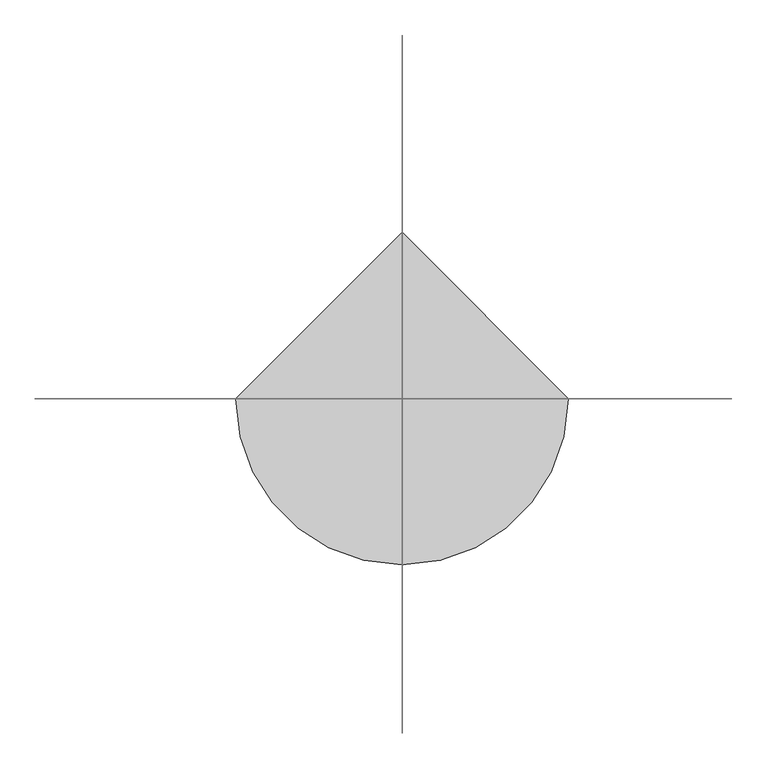
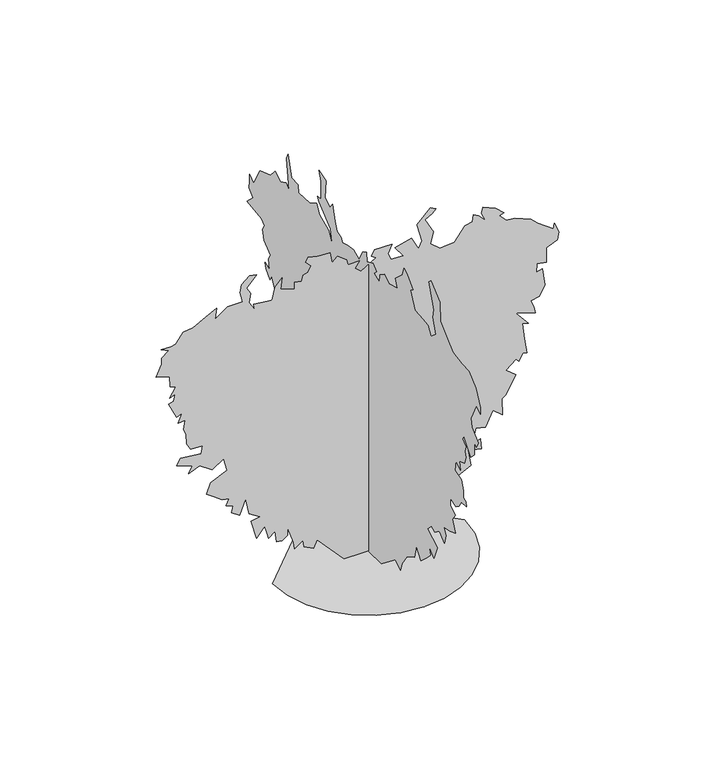
"""IFC4 building model written with IfcOpenShell, lengths in millimetres: proxy geometry, meadowlark 26084 : meadowlark 26084."""

from ifc_helpers import new_model, si_unit, origin, place, context, project, spatial, triangles, source, transform, mapped, element, save


def entourage_9ef344a8(model_context):
    return source(origin(), model_context, "Body", "Tessellation", [
        triangles([(-63.9369313, 2.6e-06, 2.5813025), (-98.6351404, 1.9e-06, 41.3616468), (-133.3335948, 1.1e-06, 80.1421467), (-143.538813, 2.7e-06, 59.7314513), (-168.0315495, 3.1e-06, 71.9778149), (-170.0726858, 2.1e-06, 90.347365), (-192.5245312, 3.9e-06, 76.0598514), (-194.5656857, 2.9e-06, 94.4296558), (-210.8940858, 9e-07, 139.3333375), (-210.8940858, 2.1e-06, 118.9223832), (-225.1818402, 3.4e-06, 108.7171649), (-239.469104, 3.9e-06, 110.7583103), (-243.5513948, 2.2e-06, 141.3742286), (-260.2917792, 3.7e-06, 128.4682213), (-264.2033864, 3e-06, 143.1357217), (-270.0860397, 2e-06, 163.8260649), (-290.4949502, 4.4e-06, 139.3333375), (-304.7824684, 2e-06, 190.3599468), (-282.331386, 8e-07, 194.4422376), (-310.9064223, 9e-07, 212.8117922), (-319.0699865, -1.4e-06, 257.7162279), (-335.3996584, 1.7e-06, 216.894083), (-355.8110942, 1.8e-06, 231.181583), (-351.7293303, 5e-07, 249.5511376), (-370.0986305, 9e-07, 255.674056), (-361.9325229, -4e-07, 272.003746), (-380.3043303, 2e-07, 276.0855281), (-401.9400736, 2e-07, 291.703997), (-421.1247311, 3e-07, 304.6605463), (-410.918995, -1.9e-06, 333.2355826), (-368.1987102, -4.9e-06, 351.9401459), (-376.2200229, -6.6e-06, 386.3038187), (-406.8371947, -4.1e-06, 367.9345184), (-439.493995, -4.1e-06, 390.385619), (-468.0690313, -2.1e-06, 378.137711), (-457.8632953, -3.5e-06, 394.4673829), (-498.6862032, -2.7e-06, 410.7970548), (-488.4805035, -4.1e-06, 427.1242195), (-435.4122311, -6.1e-06, 421.0002474), (-431.3304308, -7.5e-06, 441.4117195), (-461.9450955, -6.2e-06, 443.4538914), (-472.1508316, -6.9e-06, 461.8231553), (-474.1929671, -8.4e-06, 488.3560198), (-480.3169393, -9e-06, 502.6435561), (-476.2325955, -1.06e-05, 527.1367922), (-495.4832737, -9.7e-06, 526.35192), (-484.3987032, -1.16e-05, 549.5878564), (-498.6862032, -1.06e-05, 543.466464), (-519.0951319, -1.23e-05, 586.3290004), (-506.8497674, -1.3e-05, 590.4107643), (-502.7680035, -1.43e-05, 608.7800646), (-517.0555035, -1.33e-05, 602.6561288), (-500.7258316, -1.55e-05, 627.1493649), (-516.1995237, -1.52e-05, 634.2689884), (-517.0555035, -1.68e-05, 661.848337), (-551.7544756, -1.59e-05, 672.0540367), (-537.4644321, -1.84e-05, 702.6687378), (-538.1857907, -1.94e-05, 720.3319038), (-519.0951319, -2.1e-05, 733.2859097), (-539.506604, -2.07e-05, 743.4916094), (-512.7375257, -2.18e-05, 742.0895147), (-500.7258316, -2.25e-05, 745.5312378), (-482.3565313, -2.49e-05, 772.0666094), (-455.8236669, -2.62e-05, 774.1062378), (-423.1668666, -2.87e-05, 792.4755381), (-395.1176339, -3.08e-05, 806.3871162), (-398.6736305, -2.9e-05, 778.1880381), (-366.0168303, -3.17e-05, 800.6416821), (-327.2360942, -3.34e-05, 800.6416821), (-334.4166515, -3.47e-05, 827.9339842), (-330.1088113, -3.62e-05, 849.0616917), (-308.8667939, -3.81e-05, 865.9552826), (-290.4949502, -3.87e-05, 861.8734823), (-317.5358142, -3.58e-05, 834.0731443), (-306.8246221, -3.53e-05, 816.9688105), (-310.9064223, -3.36e-05, 792.4755381), (-296.6189042, -3.29e-05, 770.0245102), (-298.6610579, -3.37e-05, 784.3120102), (-251.0357672, -3.54e-05, 778.383593), (-243.5513948, -3.77e-05, 810.8473818), (-225.1818402, -3.97e-05, 831.2563105), (-228.2958943, -3.78e-05, 801.312208), (-192.5245312, -3.86e-05, 788.3937378), (-192.5245312, -3.97e-05, 806.7630381), (-173.5245645, -4.03e-05, 803.1613684), (-170.0726858, -4.14e-05, 819.0109823), (-157.8260678, -4.22e-05, 823.0927099), (-149.662004, -4.34e-05, 837.3802826), (-163.9495131, -4.36e-05, 851.6677826), (-157.8260678, -4.46e-05, 863.9131107), (-131.292195, -4.54e-05, 857.7916821), (-100.6760314, -4.66e-05, 855.7495102), (-94.5528496, -4.52e-05, 827.1745102), (-80.2653314, -4.65e-05, 839.4223818), (-56.9158573, -4.65e-05, 821.1673914), (-53.7314587, -4.57e-05, 806.7630381), (-23.1153655, -4.71e-05, 806.7630381), (-35.3616542, -4.56e-05, 790.4359097), (-19.0331746, -4.54e-05, 776.1484097), (19.7470164, -4.86e-05, 800.6416821), (7.5007532, -4.85e-05, 808.8052099), (15.1231208, -4.98e-05, 823.890263), (60.5683824, -5.17e-05, 823.0927099), (50.5958261, -4.99e-05, 799.816151), (58.5274868, -4.92e-05, 782.2723818), (91.1845505, -5.05e-05, 780.2302099), (68.732964, -5.13e-05, 810.8473818), (111.5952414, -5.38e-05, 821.0506107), (129.9650504, -5.25e-05, 786.3541821), (138.9452253, -5.4e-05, 804.6625122), (125.8830048, -5.64e-05, 853.7099545), (160.581223, -6e-05, 888.4063831), (174.868723, -6.01e-05, 880.2427826), (164.6635138, -5.91e-05, 870.0370829), (146.2937048, -5.76e-05, 859.8313105), (168.7455503, -5.62e-05, 819.0109823), (161.0930195, -5.4e-05, 788.6985884), (185.0742047, -5.39e-05, 767.9848818), (203.4434868, -5.48e-05, 770.0245102), (223.8544503, -5.58e-05, 772.0666094), (250.3885683, -5.9e-05, 806.7630381), (269.7101179, -6.01e-05, 811.2766434), (272.8393963, -6.13e-05, 829.2166821), (285.0872861, -6.15e-05, 823.0927099), (304.0839645, -6.12e-05, 803.1613684), (293.2508503, -6.21e-05, 827.1745102), (297.3326324, -6.31e-05, 841.4620102), (329.9894508, -6.37e-05, 827.1745102), (351.394031, -6.35e-05, 807.9441433), (340.0529354, -6.27e-05, 803.4457987), (358.5644508, -6.24e-05, 784.3120102), (381.0180948, -6.33e-05, 782.2723818), (422.1051581, -6.41e-05, 765.7470823), (440.2077596, -6.38e-05, 747.5734097), (481.0306675, -6.39e-05, 718.9984097), (483.0702959, -6.48e-05, 733.2859097), (495.3181675, -6.36e-05, 704.710837), (491.2364036, -6.23e-05, 684.2994375), (462.6588238, -6.03e-05, 672.0540367), (462.6588238, -5.8e-05, 633.273337), (438.1681312, -5.71e-05, 637.3550646), (436.1259593, -5.57e-05, 614.9040367), (452.4556312, -5.67e-05, 618.9857643), (458.5770598, -5.41e-05, 572.041464), (444.2895235, -5.19e-05, 545.5060925), (421.8384593, -5.07e-05, 541.4242922), (430.0020235, -4.98e-05, 521.0128201), (434.0863309, -4.91e-05, 504.6856916), (383.0577232, -4.78e-05, 521.0128201), (415.7145235, -4.69e-05, 482.2346274), (399.3873951, -4.64e-05, 486.3163914), (405.5087874, -4.42e-05, 443.4538914), (411.6327232, -4.2e-05, 402.6309471), (401.4269872, -4.17e-05, 404.673119), (391.2212874, -4.01e-05, 386.3038187), (383.0577232, -4.03e-05, 394.4673829), (356.5248588, -3.79e-05, 374.0559471), (383.0577232, -3.77e-05, 351.6048466), (356.5248588, -3.39e-05, 306.7001747), (346.3191227, -3.29e-05, 298.5365923), (348.3587511, -3.03e-05, 253.6334284), (323.4463909, -3.05e-05, 274.9933165), (303.4565864, -2.73e-05, 235.2636194), (278.9633503, -2.66e-05, 241.3868104), (266.8272088, -2.35e-05, 199.2829668), (291.2086966, -2.52e-05, 208.7297557), (293.2508503, -2.36e-05, 180.1547194), (258.5518782, -2.25e-05, 188.3190466), (266.7179858, -2.02e-05, 143.415374), (232.0187775, -1.77e-05, 127.0867195), (215.6903774, -1.54e-05, 100.5528377), (197.3205684, -1.5e-05, 106.6760195), (191.1973775, -1.2e-05, 61.7723423), (176.9098775, -1.3e-05, 88.306474), (150.3759956, -8.8e-06, 37.2796104), (132.0059414, -8.8e-06, 51.5671195), (68.732964, -3.2e-06, 2.5813025), (5e-07, 58.5086925, 0.0), (5.6e-06, 119.7410287, 55.1089), (6.1e-06, 137.5863239, 49.658565), (5.6e-06, 170.7679014, 104.0948725), (5.5e-06, 180.9731106, 91.8482545), (9.8e-06, 197.3017651, 73.4787044), (6.8e-06, 213.6304195, 87.7662181), (6.7e-06, 205.4660923, 93.8893999), (9.7e-06, 223.8356469, 144.9162635), (8.6e-06, 231.9999742, 112.2589454), (1e-05, 238.1231651, 136.7519272), (1.13e-05, 276.9033925, 128.5875999), (1.12e-05, 254.4523283, 148.9982999), (1.22e-05, 274.8637822, 151.0394453), (1.45e-05, 307.5205825, 171.4501453), (1.42e-05, 280.9851927, 191.8608363), (1.68e-05, 299.3544748, 232.6824725), (1.68e-05, 317.7263186, 214.3126635), (1.89e-05, 350.3043809, 228.0708535), (1.99e-05, 340.1773828, 261.2569819), (2.07e-05, 354.4649191, 265.338764), (2.22e-05, 356.5045112, 297.9955825), (2.36e-05, 393.2456552, 293.9138004), (2.61e-05, 411.6149554, 332.6945546), (2.58e-05, 397.3274554, 338.8184904), (2.92e-05, 438.1478199, 377.5992265), (2.82e-05, 405.4910196, 385.7627907), (2.9e-05, 411.6149554, 398.0081552), (2.55e-05, 417.7363478, 412.2956552), (2.48e-05, 395.2852836, 418.4196273), (2.73e-05, 415.6967194, 455.1581915), (2.98e-05, 436.1081915, 491.8993355), (2.95e-05, 444.2717557, 477.6118355), (3.11e-05, 460.5988841, 498.0207278), (3.2e-05, 466.7228199, 512.3082642), (3.07e-05, 446.3113841, 504.1447), (3.21e-05, 450.3956915, 530.6800715), (3.24e-05, 440.1899554, 547.0072), (3.47e-05, 470.8046202, 569.4583005), (3.61e-05, 476.928556, 595.9937084), (3.64e-05, 468.7649918, 610.2812084), (3.74e-05, 481.0103562, 622.5265366), (4.07e-05, 546.3265002, 630.6926805), (4.07e-05, 519.7910923, 657.2255087), (4.22e-05, 538.1603926, 673.5551805), (4.29e-05, 536.5677936, 692.1911797), (4.37e-05, 535.3943187, 712.0133709), (4.23e-05, 517.7489204, 698.0459095), (3.89e-05, 487.134292, 751.1141819), (3.76e-05, 440.1899554, 767.4438538), (3.77e-05, 419.7785196, 789.8948816), (3.6e-05, 395.2852836, 775.6073816), (3.55e-05, 370.7920475, 787.8553259), (3.44e-05, 358.546683, 775.6073816), (3.84e-05, 368.7524191, 857.250654), (3.88e-05, 362.6284833, 871.5382267), (3.56e-05, 346.2988114, 816.4303259), (3.43e-05, 317.7237751, 814.388154), (3.33e-05, 315.6841467, 793.9766819), (3.12e-05, 262.6158925, 798.0584822), (3.06e-05, 234.0411286, 814.388154), (2.9e-05, 219.7536105, 791.9370535), (2.65e-05, 180.9731106, 773.5677532), (2.43e-05, 162.603556, 740.9084095), (2.65e-05, 170.7679014, 783.7709822), (3.06e-05, 223.8356469, 824.5938538), (3.15e-05, 229.9590922, 836.8392546), (3.08e-05, 213.6301652, 838.8814264), (3.3e-05, 213.6301652, 887.8678986), (3.45e-05, 223.8356469, 912.3585548), (3.26e-05, 191.1785923, 902.1553986), (3.06e-05, 195.2606287, 853.1689264), (2.91e-05, 172.8087833, 840.9209822), (2.93e-05, 162.603556, 855.2085548), (2.71e-05, 150.356947, 816.4303259), (2.57e-05, 142.1926198, 793.9766819), (2.47e-05, 123.8230652, 787.8553259), (2.4e-05, 117.7001377, 777.6495535), (2.32e-05, 95.248047, 783.7709822), (2.23e-05, 68.7141651, 787.8553259), (2.06e-05, 43.1368564, 776.3617687), (2.13e-05, 25.8518877, 808.2641819), (2.09e-05, 9.5229755, 816.4303259), (1.98e-05, 7.4819061, 791.9370535), (1.91e-05, -19.0520211, 804.1824543), (1.78e-05, -35.3804508, 789.8948816), (1.78e-05, -25.1750781, 779.6891819), (1.63e-05, -49.6682165, 769.4834822), (1.72e-05, -51.7091075, 791.9370535), (1.69e-05, -72.1200574, 806.2245535), (1.54e-05, -92.5307528, 791.9370535), (1.42e-05, -129.2700982, 802.1428259), (1.56e-05, -121.105771, 824.5938538), (1.54e-05, -153.0015985, 852.691412), (1.61e-05, -159.8860075, 875.6199543), (1.52e-05, -172.1326437, 867.4564264), (1.28e-05, -200.7076618, 840.9209822), (1.3e-05, -188.4607894, 832.7574543), (1.02e-05, -208.8717347, 789.8948816), (8.5e-06, -245.6110801, 787.8553259), (7.4e-06, -268.0641973, 783.7709822), (5.8e-06, -280.3095436, 761.3198816), (5.7e-06, -303.1314609, 780.7331589), (8e-06, -290.5152796, 820.5121262), (8.8e-06, -294.5970617, 842.963154), (1.25e-05, -272.1459794, 906.2371988), (1.25e-05, -280.3095436, 914.4007267), (9.2e-06, -321.1299262, 879.7017546), (6.9e-06, -323.1720617, 828.675654), (4.3e-06, -354.6452497, 799.5291046), (2.2e-06, -380.3221344, 777.6495535), (1e-07, -421.1424989, 771.5255814), (-1.3e-06, -451.7596707, 769.4834822), (-3.9e-06, -482.3768789, 740.9084095), (-6.6e-06, -502.7857713, 700.0880814), (-7.4e-06, -502.7857713, 681.7187811), (-6e-06, -486.4586429, 696.0062811), (-2.7e-06, -459.9232349, 644.9801805), (-3.9e-06, -466.0472071, 624.5687084), (-6.3e-06, -494.6222071, 598.0333005), (-6.6e-06, -486.4586429, 581.7061721), (-5.9e-06, -476.2529068, 587.8301442), (-7.3e-06, -476.2529068, 555.1708005), (-7.3e-06, -459.9232349, 538.8436357), (-4.3e-06, -429.3086065, 577.6244081), (-4.5e-06, -423.1846707, 567.4186721), (-5.7e-06, -439.5143426, 555.1708005), (-6.2e-06, -433.3903705, 538.8436357), (-7.1e-06, -439.5143426, 524.5561357), (-7.6e-06, -431.3482349, 504.1447), (-7e-06, -408.8971344, 495.9810994), (-8.2e-06, -412.9789347, 473.5300352), (-6.6e-06, -392.5674625, 487.8175352), (-7.7e-06, -388.4856986, 459.2425352), (-9.4e-06, -419.1028705, 451.0764276), (-1.08e-05, -427.2664347, 426.5831915), (-1.17e-05, -428.2418112, 408.450105), (-1.23e-05, -437.4721707, 402.0924989), (-1.3e-05, -441.553971, 391.8867628), (-1.21e-05, -419.1028705, 389.844591), (-1.23e-05, -406.8549989, 371.4752907), (-1.22e-05, -394.6096344, 363.3117265), (-1.07e-05, -368.0767699, 369.4331188), (-7.3e-06, -368.0767699, 349.0242265), (-8.8e-06, -390.5278705, 336.7763186), (-9e-06, -378.2799625, 318.4070183), (-1.09e-05, -390.5278705, 287.7923899), (-1.03e-05, -366.0345981, 277.5866538), (-9.3e-06, -339.5017336, 273.5048717), (-1.05e-05, -347.6653341, 255.1330462), (-1.13e-05, -341.541362, 230.6413362), (-9.5e-06, -319.0902978, 249.0108726), (-9.2e-06, -298.6788438, 234.7233726), (-8.2e-06, -284.3913257, 242.8876998), (-8.2e-06, -266.0220254, 224.5181452), (-1.13e-05, -310.9241901, 200.0251635), (-1.22e-05, -294.5970617, 161.2446636), (-1.04e-05, -272.1459794, 181.6556089), (-1.16e-05, -278.2673899, 159.2037635), (-1.17e-05, -263.9798717, 142.8751181), (-1.15e-05, -235.4058709, 118.3821273), (-9.5e-06, -214.9951618, 144.9162635), (-1.06e-05, -205.8577653, 109.83274), (-1e-05, -174.1735256, 91.8482545), (-1.05e-05, -149.6807982, 57.1500454), (-6.7e-06, -143.5573621, 36.7393522), (-5.1e-06, -121.105771, 51.0268636), (-4.5e-06, -57.8322894, 2.0410923), (-249.8274834, 0.0, 0.0911396), (-243.2227266, -57.2440259, 0.0911358), (-224.4129918, -109.8131736, 0.091132), (-194.9037465, -156.2020027, 0.0911279), (-156.2020027, -194.9037465, 0.0911238), (-109.8131736, -224.4127374, 0.09112), (-57.2437715, -243.2227266, 0.0911167), (8.9e-06, -249.8274834, 0.0911137), (57.2440259, -243.2227266, 0.0911116), (109.8131736, -224.4127374, 0.0911454), (156.2020027, -194.9037465, 0.0911452), (194.9040008, -156.2020027, 0.0911459), (224.4127374, -109.8131736, 0.0911122), (243.2227266, -57.2437715, 0.0911147), (249.8274834, 2.18e-05, 0.0911177), (-3.49e-05, 249.8274834, 0.0911434)], [[59, 60, 61], [135, 136, 137], [51, 52, 53], [34, 35, 36], [149, 150, 151], [80, 81, 82], [172, 173, 174], [160, 161, 162], [96, 97, 98], [16, 17, 18], [16, 18, 19], [65, 66, 67], [147, 148, 149], [72, 73, 74], [71, 72, 74], [70, 71, 74], [45, 46, 47], [128, 129, 130], [6, 7, 8], [106, 107, 108], [106, 108, 109], [13, 14, 15], [102, 103, 104], [146, 147, 149], [152, 153, 154], [79, 80, 82], [166, 167, 168], [165, 166, 168], [122, 123, 124], [154, 155, 156], [112, 113, 114], [111, 112, 114], [111, 114, 115], [77, 78, 79], [21, 22, 23], [21, 23, 24], [83, 84, 85], [174, 175, 176], [36, 37, 38], [36, 38, 39], [34, 36, 39], [139, 140, 141], [55, 56, 57], [24, 25, 26], [126, 127, 128], [125, 126, 128], [125, 128, 130], [101, 102, 104], [100, 101, 104], [48, 49, 50], [47, 48, 50], [142, 143, 144], [3, 4, 5], [3, 5, 6], [110, 111, 115], [110, 115, 116], [110, 116, 117], [109, 110, 117], [69, 70, 74], [69, 74, 75], [69, 75, 76], [122, 124, 125], [157, 158, 159], [21, 24, 26], [93, 94, 95], [162, 163, 164], [170, 171, 172], [89, 90, 91], [88, 89, 91], [28, 29, 30], [28, 30, 31], [27, 28, 31], [26, 27, 31], [168, 169, 170], [11, 12, 13], [10, 11, 13], [9, 10, 13], [91, 92, 93], [88, 91, 93], [87, 88, 93], [13, 15, 16], [93, 95, 96], [21, 26, 31], [32, 33, 34], [32, 34, 39], [32, 39, 40], [79, 82, 83], [100, 104, 105], [53, 54, 55], [6, 8, 9], [64, 65, 67], [85, 86, 87], [57, 58, 59], [99, 100, 105], [55, 57, 59], [40, 41, 42], [40, 42, 43], [135, 137, 138], [135, 138, 139], [134, 135, 139], [142, 144, 145], [142, 145, 146], [152, 154, 156], [134, 139, 141], [157, 159, 160], [142, 146, 149], [62, 63, 64], [177, 1, 2], [176, 177, 2], [176, 2, 3], [85, 87, 93], [19, 20, 21], [125, 130, 131], [133, 134, 141], [132, 133, 141], [131, 132, 141], [174, 176, 3], [109, 117, 118], [85, 93, 96], [85, 96, 98], [83, 85, 98], [125, 131, 141], [125, 141, 142], [125, 142, 149], [122, 125, 149], [121, 122, 149], [120, 121, 149], [119, 120, 149], [118, 119, 149], [83, 98, 99], [47, 50, 51], [172, 174, 3], [59, 61, 62], [55, 59, 62], [55, 62, 64], [55, 64, 67], [53, 55, 67], [9, 13, 16], [9, 16, 19], [157, 160, 162], [168, 170, 172], [168, 172, 3], [165, 168, 3], [164, 165, 3], [164, 3, 6], [164, 6, 9], [164, 9, 19], [164, 19, 21], [164, 21, 31], [164, 31, 32], [162, 164, 32], [157, 162, 32], [157, 32, 40], [157, 40, 43], [157, 43, 44], [157, 44, 45], [157, 45, 47], [157, 47, 51], [157, 51, 53], [157, 53, 67], [157, 67, 68], [156, 157, 68], [152, 156, 68], [109, 118, 149], [106, 109, 149], [105, 106, 149], [99, 105, 149], [99, 149, 151], [99, 151, 152], [83, 99, 152], [79, 83, 152], [77, 79, 152], [77, 152, 68], [77, 68, 69], [76, 77, 69], [186, 187, 188], [188, 189, 190], [232, 233, 234], [231, 232, 234], [308, 309, 310], [211, 212, 213], [292, 293, 294], [246, 247, 248], [219, 220, 221], [246, 248, 249], [245, 246, 249], [250, 251, 252], [223, 224, 225], [202, 203, 204], [327, 328, 329], [259, 260, 261], [209, 210, 211], [209, 211, 213], [191, 192, 193], [243, 244, 245], [333, 334, 335], [332, 333, 335], [271, 272, 273], [315, 316, 317], [314, 315, 317], [342, 343, 344], [273, 274, 275], [258, 259, 261], [291, 292, 294], [271, 273, 275], [183, 184, 185], [182, 183, 185], [326, 327, 329], [205, 206, 207], [300, 301, 302], [299, 300, 302], [321, 322, 323], [297, 298, 299], [296, 297, 299], [262, 263, 264], [261, 262, 264], [296, 299, 302], [337, 338, 339], [200, 201, 202], [199, 200, 202], [323, 324, 325], [242, 243, 245], [242, 245, 249], [242, 249, 250], [242, 250, 252], [242, 252, 253], [237, 238, 239], [283, 284, 285], [282, 283, 285], [282, 285, 286], [281, 282, 286], [280, 281, 286], [280, 286, 287], [195, 196, 197], [194, 195, 197], [241, 242, 253], [241, 253, 254], [241, 254, 255], [234, 235, 236], [231, 234, 236], [227, 228, 229], [190, 191, 193], [179, 180, 181], [303, 304, 305], [229, 230, 231], [270, 271, 275], [269, 270, 275], [269, 275, 276], [197, 198, 199], [266, 267, 268], [265, 266, 268], [222, 223, 225], [221, 222, 225], [186, 188, 190], [182, 185, 186], [181, 182, 186], [204, 205, 207], [329, 330, 331], [323, 325, 326], [280, 287, 288], [321, 323, 326], [311, 312, 313], [335, 336, 337], [335, 337, 339], [332, 335, 339], [295, 296, 302], [277, 278, 279], [219, 221, 225], [219, 225, 226], [219, 226, 227], [219, 227, 229], [218, 219, 229], [218, 229, 231], [186, 190, 193], [306, 307, 308], [305, 306, 308], [303, 305, 308], [303, 308, 310], [311, 313, 314], [311, 314, 317], [311, 317, 318], [311, 318, 319], [311, 319, 320], [339, 340, 341], [258, 261, 264], [345, 178, 179], [344, 345, 179], [344, 179, 181], [216, 217, 218], [215, 216, 218], [215, 218, 231], [215, 231, 236], [215, 236, 237], [215, 237, 239], [215, 239, 240], [215, 240, 241], [341, 342, 344], [341, 344, 181], [339, 341, 181], [332, 339, 181], [332, 181, 186], [332, 186, 193], [332, 193, 194], [331, 332, 194], [279, 280, 288], [290, 291, 294], [289, 290, 294], [289, 294, 295], [288, 289, 295], [279, 288, 295], [279, 295, 302], [279, 302, 303], [279, 303, 310], [213, 214, 215], [209, 213, 215], [209, 215, 241], [208, 209, 241], [207, 208, 241], [326, 329, 331], [321, 326, 331], [321, 331, 194], [320, 321, 194], [311, 320, 194], [310, 311, 194], [279, 310, 194], [277, 279, 194], [276, 277, 194], [269, 276, 194], [268, 269, 194], [265, 268, 194], [264, 265, 194], [258, 264, 194], [258, 194, 197], [258, 197, 199], [258, 199, 202], [258, 202, 204], [258, 204, 207], [258, 207, 241], [258, 241, 255], [258, 255, 256], [257, 258, 256], [360, 361, 346], [359, 360, 346], [359, 346, 347], [358, 359, 347], [358, 347, 348], [358, 348, 349], [357, 358, 349], [356, 357, 349], [356, 349, 350], [356, 350, 351], [356, 351, 352], [356, 352, 353], [356, 353, 354], [356, 354, 355]], closed=False),
    ])


if __name__ == "__main__":
    model = new_model("IFC4")
    model_context = context("Model", 3, world=origin())
    ifc_project = project(units=[si_unit("LENGTHUNIT", "METRE", prefix="MILLI")], contexts=[model_context])
    site = spatial("IfcSite", under=ifc_project)
    building = spatial("IfcBuilding", under=site)
    placement = place(None, origin())
    entourage_shape = entourage_9ef344a8(model_context)
    element("IfcBuildingElementProxy", 1, Name="meadowlark 26084 : meadowlark 26084", ObjectType="meadowlark 26084 : meadowlark 26084", at=placement, inside=building, context=model_context, shape_type="MappedRepresentation", body=[
        mapped(entourage_shape, transform((0.0, 0.0, 0.0), x_axis=(1.0, 0.0, 0.0), y_axis=(0.0, 1.0, 0.0), z_axis=(0.0, 0.0, 1.0))),
    ])
    save(model, "model.ifc")

# Revit data of these elements
# Type "meadowlark 26084 : meadowlark 26084"
#   built-in parameter 1005195 = "RPC-16-G0FT-Q7G0-0DUH-W000-ST1L-LVER-AU"
#   Height = 0
